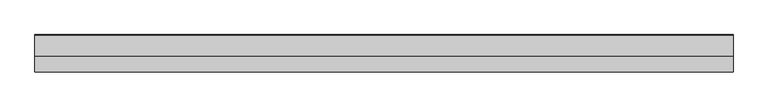
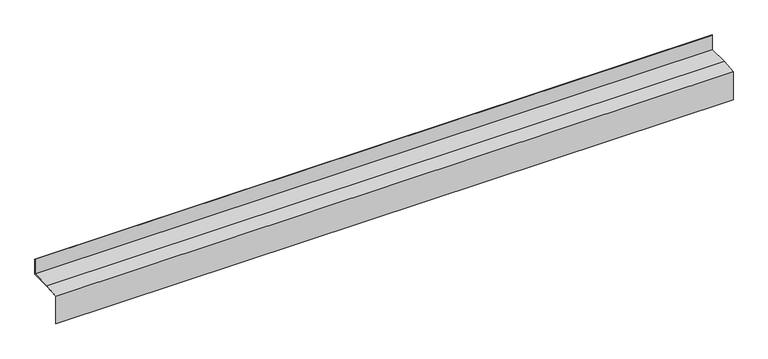
"""IFC4 building model written with IfcOpenShell, lengths in millimetres: proxy geometry, Generic Models 7:Generic Models 1:7:Generic Models 1:7 : Generic Models 7:Generic Models 1:337419:7 : Generic Models 7:Generic Models 1:7:Generic Models 1:7 : Generic Models 7:Generic Models 1:337419:315055."""

from ifc_helpers import new_model, si_unit, frame, origin, place, context, project, spatial, polyline, outline, extrude, source, transform, mapped, element, save


def generic_models_35fec10c(model_context):
    return source(origin(), model_context, "Body", "SweptSolid", [
        extrude(outline(polyline([(-579143.2285706, -81.7582633), (-579144.8160706, -81.7582633), (-579144.8160706, 24.2909738), (-579089.3872692, 30.4457208), (-579015.3287878, 30.4457208), (-579015.3287878, 85.7752465), (-579013.7412878, 85.7752465), (-579013.7412878, 28.8582208), (-579089.2994022, 28.8582208), (-579143.2285706, 22.8699913), (-579143.2285706, -81.7582633)])), frame((593738.0867239, 0.0, 0.0), z_axis=(1.0, 0.0, 0.0), x_axis=(0.0, 1.0, 0.0)), (0.0, 0.0, 1.0), 2447.788191),
    ])


if __name__ == "__main__":
    model = new_model("IFC4")
    model_context = context("Model", 3, world=origin())
    ifc_project = project(units=[si_unit("LENGTHUNIT", "METRE", prefix="MILLI")], contexts=[model_context])
    site = spatial("IfcSite", under=ifc_project)
    building = spatial("IfcBuilding", under=site)
    placement = place(None, origin())
    generic_models_shape = generic_models_35fec10c(model_context)
    element("IfcBuildingElementProxy", 1, Name="Generic Models 7:Generic Models 1:7:Generic Models 1:7 : Generic Models 7:Generic Models 1:337419:7 : Generic Models 7:Generic Models 1:7:Generic Models 1:7 : Generic Models 7:Generic Models 1:337419:315055", ObjectType="Generic Models 7:Generic Models 1:7:Generic Models 1:7 : Generic Models 7:Generic Models 1:337419:7 : Generic Models 7:Generic Models 1:7:Generic Models 1:7 : Generic Models 7:Generic Models 1:337419:315055", at=placement, inside=building, context=model_context, shape_type="MappedRepresentation", body=[
        mapped(generic_models_shape, transform((0.0, 0.0, 0.0), x_axis=(1.0, 0.0, 0.0), y_axis=(0.0, 1.0, 0.0), z_axis=(0.0, 0.0, 1.0))),
    ])
    save(model, "model.ifc")

# Revit data of these elements
# Type "Generic Models 7:Generic Models 1:7:Generic Models 1:7 : Generic Models 7:Generic Models 1:337419:7 : Generic Models 7:Generic Models 1:7:Generic Models 1:7 : Generic Models 7:Generic Models 1:337419:315055"
#   NameOverride = "Generic Models 7:Generic Models 1:7:Generic Models 1:7 : Generic Models 7:Generic Models 1:337419:315055"
#   ObjectTypeOverride = "Generic Models 1:7 : Generic Models 7:Generic Models 1:337419"
#   Reference = "Generic Models 1"
#   Tag = "315055"
# Element 1 (IfcBuildingElementProxy, "Generic Models 7:Generic Models 1:7:Generic Models 1:7 : Generic Models 7:Generic Models 1:337419:7 : Generic Models 7:Generic Models 1:7:Generic Models 1:7 : Generic Models 7:Generic Models 1:337419:315055")
#   Materials on its faces: "ANODIZED ALUM. FLASHING - MATCH STOREFRONT (ALIGN WITH OTHER WALL ASSEMBLIES)"
# Materials
#   "ANODIZED ALUM. FLASHING - MATCH STOREFRONT (ALIGN WITH OTHER WALL ASSEMBLIES)": class "Unassigned", colour RGB 210 209 208, transparency 0, Cost = 0
